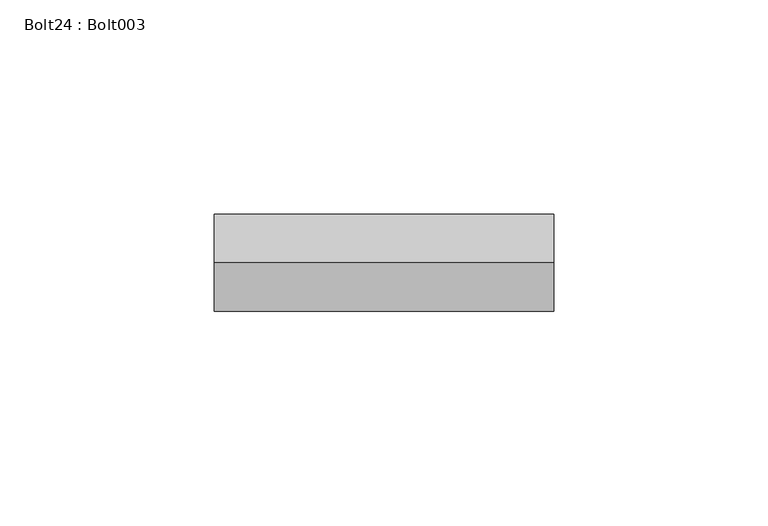
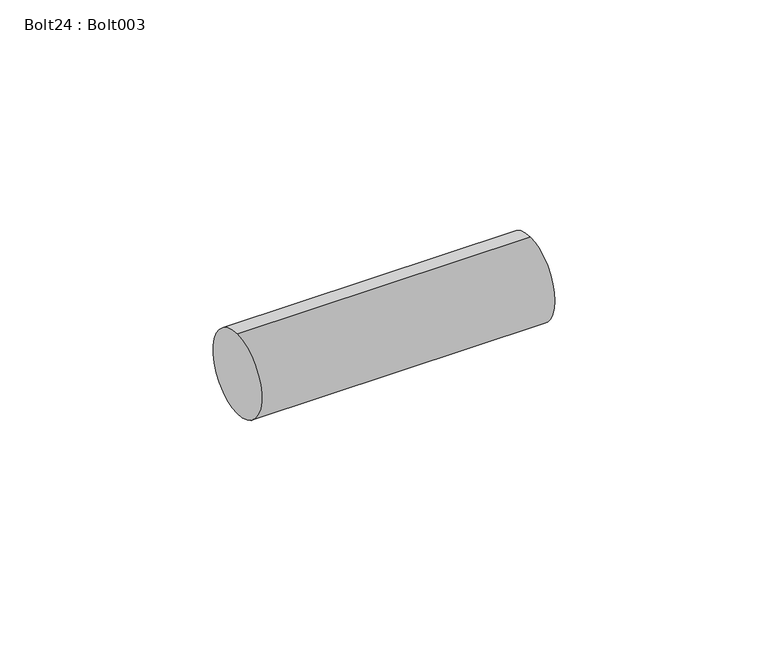
"""IFC4 building model written with IfcOpenShell, lengths in millimetres: proxy geometry, Bolt24 : Bolt003."""

from ifc_helpers import new_model, si_unit, point, frame, frame_2d, origin, place, context, project, spatial, circle_curve, trimmed, segment, composite_curve, outline, extrude, source, transform, mapped, element, save


def bolt24_bolt003_f55f5b75(model_context):
    return source(origin(), model_context, "Body", "SweptSolid", [
        extrude(outline(composite_curve([segment(trimmed(circle_curve(frame_2d((1985.8304801, 39960.0063132)), 11.4045168), [point((1985.8304801, 39971.41083))], [point((1985.8304801, 39948.6017964))], False, "CARTESIAN"), True, "CONTINUOUS"), segment(trimmed(circle_curve(frame_2d((1985.8304801, 39960.0063132)), 11.4045168), [point((1985.8304801, 39948.6017964))], [point((1985.8304801, 39971.41083))], False, "CARTESIAN"), True, "CONTINUOUS")], self_intersect=False)), frame((10265.0890809, 0.0, 0.0), z_axis=(1.0, 0.0, 0.0), x_axis=(0.0, 1.0, 0.0)), (0.0, 0.0, 1.0), 79.375),
    ])


if __name__ == "__main__":
    model = new_model("IFC4")
    model_context = context("Model", 3, world=origin())
    ifc_project = project(units=[si_unit("LENGTHUNIT", "METRE", prefix="MILLI")], contexts=[model_context])
    site = spatial("IfcSite", under=ifc_project)
    building = spatial("IfcBuilding", under=site)
    placement = place(None, origin())
    bolt24_bolt003_shape = bolt24_bolt003_f55f5b75(model_context)
    element("IfcBuildingElementProxy", 1, Name="Bolt24 : Bolt003", ObjectType="Bolt24 : Bolt003", at=placement, inside=building, context=model_context, shape_type="MappedRepresentation", body=[
        mapped(bolt24_bolt003_shape, transform((0.0, 0.0, 0.0), x_axis=(1.0, 0.0, 0.0), y_axis=(0.0, 1.0, 0.0), z_axis=(0.0, 0.0, 1.0))),
    ])
    save(model, "model.ifc")

# Revit data of these elements
# Type "Bolt24 : Bolt003"
#   NameOverride = "Bolt003"
# Element 1 (IfcBuildingElementProxy, "Bolt24 : Bolt003")
#   Materials on its faces: "TUBE STEEL STRINGER WELDED TO ANCHORED STEEL PLATE - SEE STRUCT DWGS"
# Materials
#   "TUBE STEEL STRINGER WELDED TO ANCHORED STEEL PLATE - SEE STRUCT DWGS": class "Unassigned", colour RGB 128 128 128, transparency 0, Cost = 0
